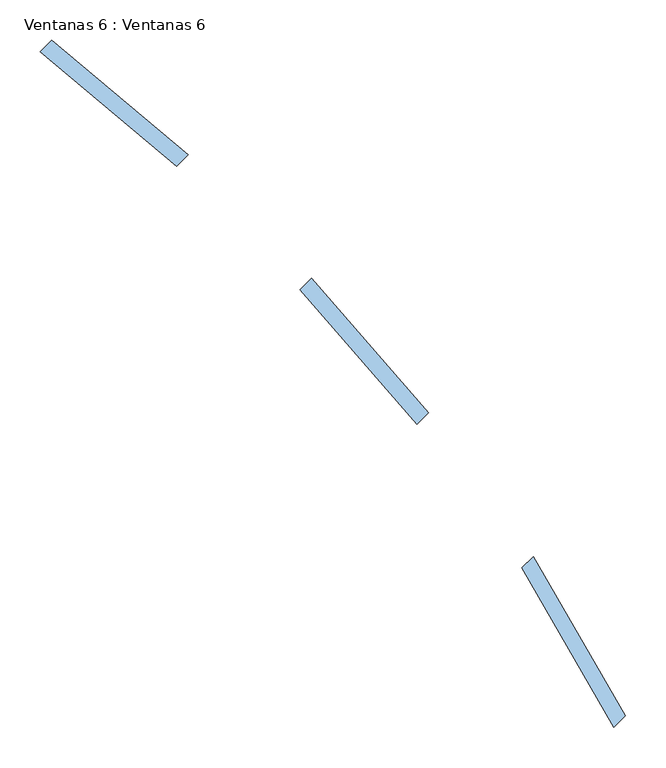
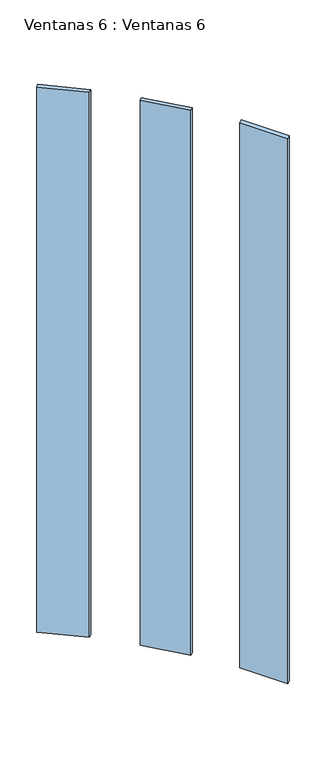
"""IFC4 building model written with IfcOpenShell, lengths in millimetres: window geometry, Ventanas 6 : Ventanas 6."""

from ifc_helpers import new_model, si_unit, frame, origin, place, context, project, spatial, polyline, outline, extrude, source, transform, mapped, element, save


def ventanas_6_ventanas_6_e0f00053(model_context):
    return source(origin(), model_context, "Body", "SweptSolid", [
        extrude(outline(polyline([(-1472.4495786, 13242.5043113), (-1486.5917142, 13228.3621757), (-1655.7652481, 13370.3156256), (-1641.6231124, 13384.4577612), (-1472.4495786, 13242.5043113)])), frame((0.0, 0.0, 6100.0), z_axis=(0.0, 0.0, 1.0), x_axis=(1.0, 0.0, 0.0)), (0.0, 0.0, 1.0), 2739.3335698),
        extrude(outline(polyline([(-1175.0228001, 12923.3214147), (-1189.1649357, 12909.1792791), (-1333.8503685, 13075.62083), (-1319.7082329, 13089.7629656), (-1175.0228001, 12923.3214147)])), frame((0.0, 0.0, 6100.0), z_axis=(0.0, 0.0, 1.0), x_axis=(1.0, 0.0, 0.0)), (0.0, 0.0, 1.0), 2739.3335698),
        extrude(outline(polyline([(-930.623735, 12547.8343766), (-944.7658706, 12533.692241), (-1058.6462505, 12730.9388449), (-1044.5041148, 12745.0809805), (-930.623735, 12547.8343766)])), frame((0.0, 0.0, 6100.0), z_axis=(0.0, 0.0, 1.0), x_axis=(1.0, 0.0, 0.0)), (0.0, 0.0, 1.0), 2739.3335698),
    ])


if __name__ == "__main__":
    model = new_model("IFC4")
    model_context = context("Model", 3, world=origin())
    ifc_project = project(units=[si_unit("LENGTHUNIT", "METRE", prefix="MILLI")], contexts=[model_context])
    site = spatial("IfcSite", under=ifc_project)
    building = spatial("IfcBuilding", under=site)
    placement = place(None, origin())
    ventanas_6_ventanas_6_shape = ventanas_6_ventanas_6_e0f00053(model_context)
    element("IfcWindow", 1, ObjectType="Ventanas 6 : Ventanas 6", at=placement, inside=building, context=model_context, shape_type="MappedRepresentation", body=[
        mapped(ventanas_6_ventanas_6_shape, transform((0.0, 0.0, 0.0), x_axis=(1.0, 0.0, 0.0), y_axis=(0.0, 1.0, 0.0), z_axis=(0.0, 0.0, 1.0))),
    ])
    save(model, "model.ifc")

# Revit data of these elements
# Type "Ventanas 6 : Ventanas 6"
#   Type Mark = "32"
# Element 1 (IfcWindow, "Ventanas 6 : Ventanas 6")
#   Materials on its faces: "VIDRIO"
# Materials
#   "VIDRIO": class "Genérico", colour RGB 120 120 120, transparency 0, Cost = 0
